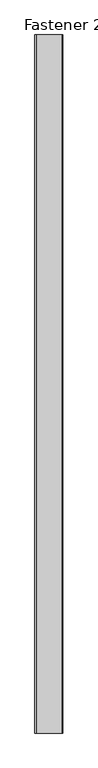
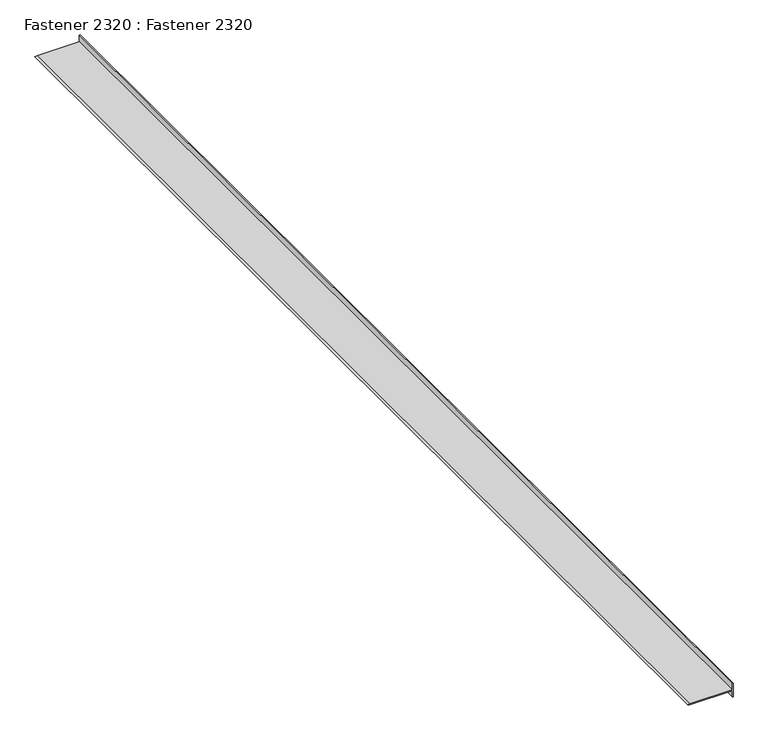
"""IFC4 building model written with IfcOpenShell, lengths in millimetres: proxy geometry, Fastener 2320 : Fastener 2320."""

from ifc_helpers import new_model, si_unit, frame, origin, place, context, project, spatial, polyline, outline, extrude, source, transform, mapped, element, save


def fastener_2320_fastener_2320_162db988(model_context):
    return source(origin(), model_context, "Body", "SweptSolid", [
        extrude(outline(polyline([(40087.9789725, -7085.0334918), (40113.3789725, -7085.0334918), (40113.3789725, -7086.4358356), (40101.3801444, -7086.4358356), (40101.3801444, -7161.2334918), (40100.6789725, -7165.0461872), (40099.9778006, -7161.2334918), (40099.9778006, -7086.4358356), (40087.9789725, -7086.4358356), (40087.9789725, -7085.0334918)])), frame((0.0, 7982.1531721, 0.0), z_axis=(0.0, 1.0, 0.0), x_axis=(0.0, 0.0, 1.0)), (0.0, 0.0, 1.0), 1999.85),
    ])


if __name__ == "__main__":
    model = new_model("IFC4")
    model_context = context("Model", 3, world=origin())
    ifc_project = project(units=[si_unit("LENGTHUNIT", "METRE", prefix="MILLI")], contexts=[model_context])
    site = spatial("IfcSite", under=ifc_project)
    building = spatial("IfcBuilding", under=site)
    placement = place(None, origin())
    fastener_2320_fastener_2320_shape = fastener_2320_fastener_2320_162db988(model_context)
    element("IfcBuildingElementProxy", 1, Name="Fastener 2320 : Fastener 2320", ObjectType="Fastener 2320 : Fastener 2320", at=placement, inside=building, context=model_context, shape_type="MappedRepresentation", body=[
        mapped(fastener_2320_fastener_2320_shape, transform((0.0, 0.0, 0.0), x_axis=(1.0, 0.0, 0.0), y_axis=(0.0, 1.0, 0.0), z_axis=(0.0, 0.0, 1.0))),
    ])
    save(model, "model.ifc")

# Revit data of these elements
# Type "Fastener 2320 : Fastener 2320"
#   NameOverride = "Fastener"
# Element 1 (IfcBuildingElementProxy, "Fastener 2320 : Fastener 2320")
#   Materials on its faces: "FASTEN INTO BLOCKING"
# Materials
#   "FASTEN INTO BLOCKING": class "Unassigned", colour RGB 255 255 255, transparency 0
